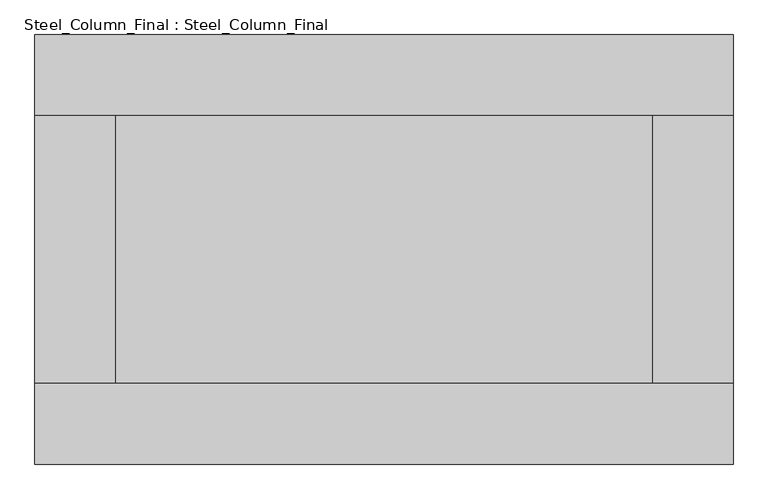
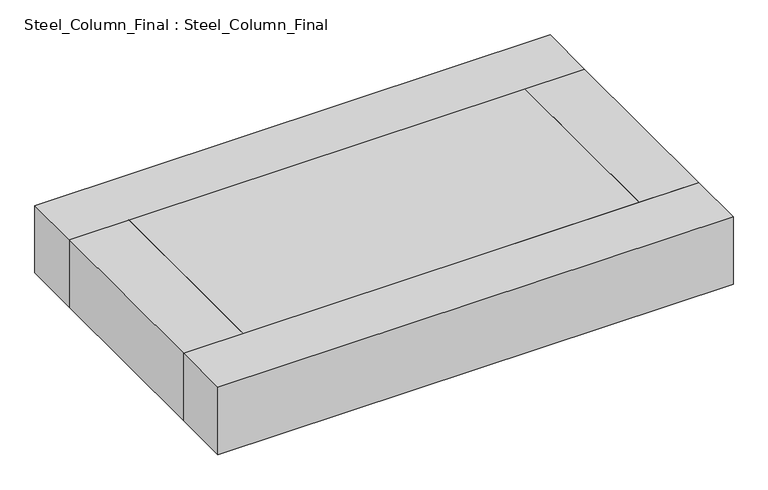
"""IFC4 building model written with IfcOpenShell, lengths in millimetres: proxy geometry, Steel_Column_Final : Steel_Column_Final."""

from ifc_helpers import new_model, si_unit, frame, origin, place, context, project, spatial, polyline, outline, extrude, source, transform, mapped, element, save


def steel_column_final_steel_column_final_49b77c8d(model_context):
    return source(origin(), model_context, "Body", "SweptSolid", [
        extrude(outline(polyline([(6500.0, 2500.0), (-6500.0, 2500.0), (-6500.0, 4000.0), (6500.0, 4000.0), (6500.0, 2500.0)])), frame((0.0, 0.0, 79290.0), z_axis=(0.0, 0.0, 1.0), x_axis=(1.0, 0.0, 0.0)), (0.0, 0.0, 1.0), 1800.0),
        extrude(outline(polyline([(-6500.0, -2500.0), (6500.0, -2500.0), (6500.0, -4000.0), (-6500.0, -4000.0), (-6500.0, -2500.0)])), frame((0.0, 0.0, 79290.0), z_axis=(0.0, 0.0, 1.0), x_axis=(1.0, 0.0, 0.0)), (0.0, 0.0, 1.0), 1800.0),
        extrude(outline(polyline([(5000.0, -2500.0), (5000.0, 2500.0), (6500.0, 2500.0), (6500.0, -2500.0), (5000.0, -2500.0)])), frame((0.0, 0.0, 79290.0), z_axis=(0.0, 0.0, 1.0), x_axis=(1.0, 0.0, 0.0)), (0.0, 0.0, 1.0), 1800.0),
        extrude(outline(polyline([(-5000.0, 2500.0), (-5000.0, -2500.0), (-6500.0, -2500.0), (-6500.0, 2500.0), (-5000.0, 2500.0)])), frame((0.0, 0.0, 79290.0), z_axis=(0.0, 0.0, 1.0), x_axis=(1.0, 0.0, 0.0)), (0.0, 0.0, 1.0), 1800.0),
        extrude(outline(polyline([(-5000.0, -2500.0), (-5000.0, 2500.0), (5000.0, 2500.0), (5000.0, -2500.0), (-5000.0, -2500.0)])), frame((0.0, 0.0, 79290.0), z_axis=(0.0, 0.0, 1.0), x_axis=(1.0, 0.0, 0.0)), (0.0, 0.0, 1.0), 1800.0),
    ])


if __name__ == "__main__":
    model = new_model("IFC4")
    model_context = context("Model", 3, world=origin())
    ifc_project = project(units=[si_unit("LENGTHUNIT", "METRE", prefix="MILLI")], contexts=[model_context])
    site = spatial("IfcSite", under=ifc_project)
    building = spatial("IfcBuilding", under=site)
    placement = place(None, origin())
    steel_column_final_steel_column_final_shape = steel_column_final_steel_column_final_49b77c8d(model_context)
    element("IfcBuildingElementProxy", 1, Name="Steel_Column_Final : Steel_Column_Final", ObjectType="Steel_Column_Final : Steel_Column_Final", at=placement, inside=building, context=model_context, shape_type="MappedRepresentation", body=[
        mapped(steel_column_final_steel_column_final_shape, transform((0.0, 0.0, 0.0), x_axis=(1.0, 0.0, 0.0), y_axis=(0.0, 1.0, 0.0), z_axis=(0.0, 0.0, 1.0))),
    ])
    save(model, "model.ifc")

# Revit data of these elements
# Type "Steel_Column_Final : Steel_Column_Final"
#   Top Width [instance default] = 5000 mm
#   Top Length = 10000 mm
#   Length = 21000 mm
#   Height [instance default] = 50000 mm
#   Bottom Width [instance default] = 5000 mm
#   Default Elevation = 0
# Element 1 (IfcBuildingElementProxy, "Steel_Column_Final : Steel_Column_Final")
#   Height = 79290 mm
